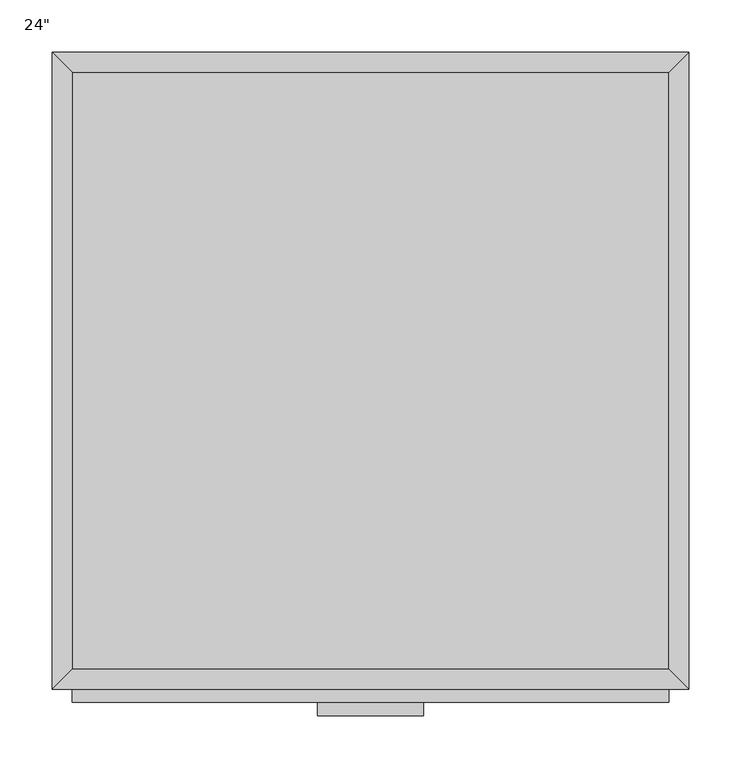
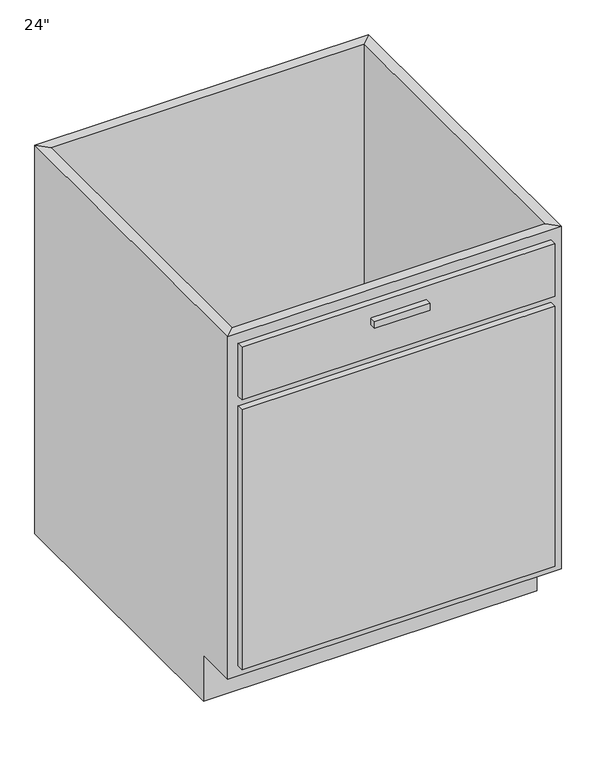
"""IFC4 building model written with IfcOpenShell, lengths in millimetres: furniture geometry."""

from ifc_helpers import new_model, si_unit, frame, origin, place, context, project, spatial, polyline, outline, extrude, faceted_brep, source, transform, mapped, element, save


def furniture_b7a4a562(model_context):
    return source(origin(), model_context, "Body", "SolidModel", [
        faceted_brep([(304.4877049, -590.55, 749.3), (304.4877049, -590.55, 88.9), (-267.0122951, -590.55, 88.9), (-267.0122951, -590.55, 749.3), (-286.0622951, -609.6, 749.3), (323.5377049, -609.6, 749.3), (-286.0622951, -609.6, 88.9), (323.5377049, -609.6, 88.9), (-267.0122951, -533.4, 88.9), (-267.0122951, -19.05, 88.9), (-267.0122951, -19.05, 749.3), (-286.0622951, 0.0, 749.3), (-286.0622951, 0.0, 0.0), (-286.0622951, -533.4, 0.0), (-286.0622951, -533.4, 88.9), (304.4877049, -19.05, 88.9), (304.4877049, -19.05, 749.3), (323.5377049, 0.0, 749.3), (323.5377049, 0.0, 0.0), (304.4877049, -533.4, 88.9), (323.5377049, -533.4, 88.9), (323.5377049, -533.4, 0.0)], [[[0, 1, 2, 3]], [[0, 3, 4, 5]], [[5, 4, 6, 7]], [[2, 1, 7, 6]], [[3, 2, 8, 9, 10]], [[4, 3, 10, 11]], [[6, 4, 11, 12, 13, 14]], [[2, 6, 14, 8]], [[10, 9, 15, 16]], [[11, 10, 16, 17]], [[12, 11, 17, 18]], [[1, 0, 16, 15, 19]], [[0, 5, 17, 16]], [[5, 7, 20, 21, 18, 17]], [[7, 1, 19, 20]], [[8, 19, 15, 9]], [[18, 21, 13, 12]], [[13, 21, 20, 19, 8, 14]]]),
        extrude(outline(polyline([(304.4877049, -19.05), (304.4877049, -590.55), (-267.0122951, -590.55), (-267.0122951, -19.05), (304.4877049, -19.05)])), frame((0.0, 0.0, 88.9), z_axis=(0.0, 0.0, 1.0), x_axis=(1.0, 0.0, 0.0)), (0.0, 0.0, 1.0), 19.05),
        extrude(outline(polyline([(304.4877049, -622.3), (-267.0122951, -622.3), (-267.0122951, -609.6), (304.4877049, -609.6), (304.4877049, -622.3)])), frame((0.0, 0.0, 628.65), z_axis=(0.0, 0.0, 1.0), x_axis=(1.0, 0.0, 0.0)), (0.0, 0.0, 1.0), 101.6),
        extrude(outline(polyline([(304.4877049, -622.3), (-267.0122951, -622.3), (-267.0122951, -609.6), (304.4877049, -609.6), (304.4877049, -622.3)])), frame((0.0, 0.0, 107.95), z_axis=(0.0, 0.0, 1.0), x_axis=(1.0, 0.0, 0.0)), (0.0, 0.0, 1.0), 501.65),
        extrude(outline(polyline([(69.5377049, -635.0), (-32.0622951, -635.0), (-32.0622951, -622.3), (69.5377049, -622.3), (69.5377049, -635.0)])), frame((0.0, 0.0, 692.15), z_axis=(0.0, 0.0, 1.0), x_axis=(1.0, 0.0, 0.0)), (0.0, 0.0, 1.0), 12.7),
    ])


if __name__ == "__main__":
    model = new_model("IFC4")
    model_context = context("Model", 3, world=origin())
    ifc_project = project(units=[si_unit("LENGTHUNIT", "METRE", prefix="MILLI")], contexts=[model_context])
    site = spatial("IfcSite", under=ifc_project)
    building = spatial("IfcBuilding", under=site)
    placement = place(None, origin())
    furniture_shape = furniture_b7a4a562(model_context)
    element("IfcFurniture", 1, ObjectType="Vanity Cabinet-Single Door & Drawer : 24\"", at=placement, inside=building, context=model_context, shape_type="MappedRepresentation", body=[
        mapped(furniture_shape, transform((0.0, 0.0, 0.0), x_axis=(1.0, 0.0, 0.0), y_axis=(0.0, 1.0, 0.0), z_axis=(0.0, 0.0, 1.0))),
    ])
    save(model, "model.ifc")

# Revit data of these elements
# Type "Vanity Cabinet-Single Door & Drawer : 24\""
#   Assembly Code = "C1030410"
#   Depth = 2' - 0"
#   Height = 2' - 5 1/2"
#   Toe Depth = 0' - 3"
#   Toe Height = 0' - 3 1/2"
#   Width = 2' - 0"
#   Cabinet Material = none
#   Door/Drawer Material = none
#   Handle Material = Cabinets - Handles
# Element 1 (IfcFurniture, "Vanity Cabinet-Single Door & Drawer : 24\"")
#   Materials on its faces: "Cabinets", "Cabinets - Handles"
# Materials
#   "Cabinets - Handles": class "Metal", colour RGB 57 57 57, transparency 0
#   "Cabinets": class "Miscellaneous", colour RGB 249 249 249, transparency 0
